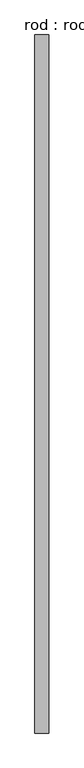
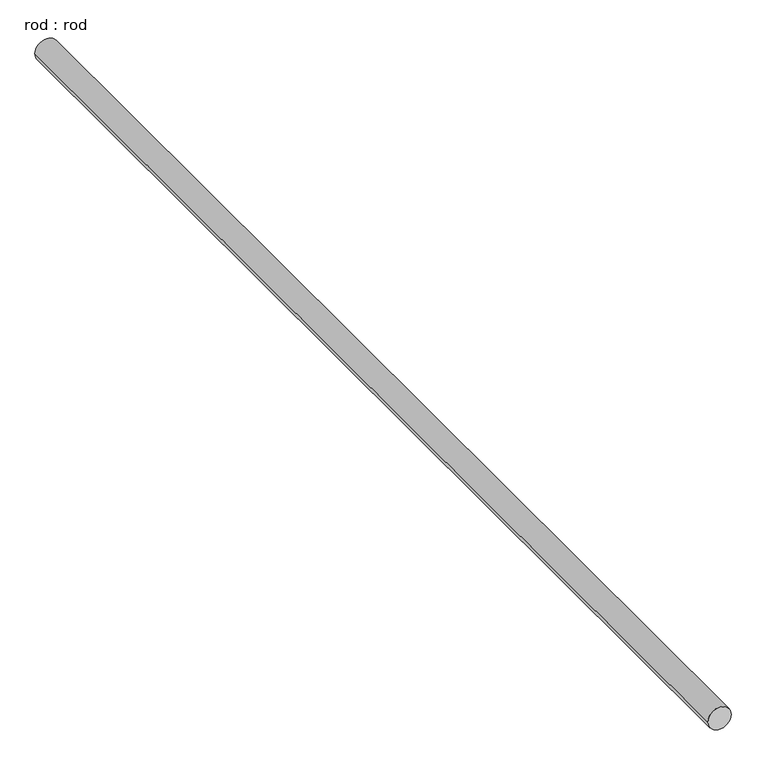
"""IFC4 building model written with IfcOpenShell, lengths in millimetres: proxy geometry, rod : rod."""

from ifc_helpers import new_model, si_unit, point, frame, frame_2d, origin, place, context, project, spatial, circle_curve, trimmed, segment, composite_curve, outline, extrude, source, transform, mapped, element, save


def rod_rod_bffb7d0c(model_context):
    return source(origin(), model_context, "Body", "SweptSolid", [
        extrude(outline(composite_curve([segment(trimmed(circle_curve(frame_2d((0.0108462, 0.0)), 200.0), [point((0.0108462, 200.0))], [point((0.0108462, -200.0))], False, "CARTESIAN"), True, "CONTINUOUS"), segment(trimmed(circle_curve(frame_2d((0.0108462, 0.0)), 200.0), [point((0.0108462, -200.0))], [point((0.0108462, 200.0))], False, "CARTESIAN"), True, "CONTINUOUS")], self_intersect=False)), frame((0.0, -5938.5213847, 0.0), z_axis=(0.0, 1.0, 0.0), x_axis=(0.0, 0.0, 1.0)), (0.0, 0.0, 1.0), 20062.5),
    ])


if __name__ == "__main__":
    model = new_model("IFC4")
    model_context = context("Model", 3, world=origin())
    ifc_project = project(units=[si_unit("LENGTHUNIT", "METRE", prefix="MILLI")], contexts=[model_context])
    site = spatial("IfcSite", under=ifc_project)
    building = spatial("IfcBuilding", under=site)
    placement = place(None, origin())
    rod_rod_shape = rod_rod_bffb7d0c(model_context)
    element("IfcBuildingElementProxy", 1, Name="rod : rod", ObjectType="rod : rod", at=placement, inside=building, context=model_context, shape_type="MappedRepresentation", body=[
        mapped(rod_rod_shape, transform((0.0, 0.0, 0.0), x_axis=(1.0, 0.0, 0.0), y_axis=(0.0, 1.0, 0.0), z_axis=(0.0, 0.0, 1.0))),
    ])
    save(model, "model.ifc")

# Revit data of these elements
# Type "rod : rod"
#   Default Elevation = 0
